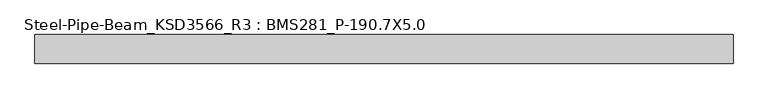
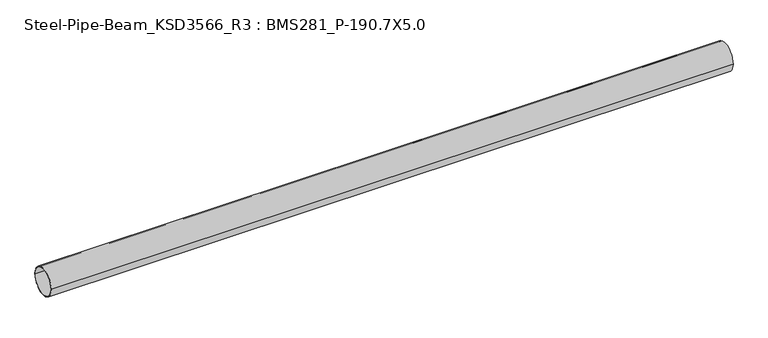
"""IFC4 building model written with IfcOpenShell, lengths in millimetres: member geometry, Steel-Pipe-Beam_KSD3566_R3 : BMS281_P-190.7X5.0."""

from ifc_helpers import new_model, si_unit, point, frame, origin, origin_2d, place, context, project, spatial, circle_curve, trimmed, segment, composite_curve, outline, extrude, source, transform, mapped, element, save


def steel_pipe_beam_ksd3566_r3_bms281_p_190_7x5_0_96b81fe0(model_context):
    return source(origin(), model_context, "Body", "SweptSolid", [
        extrude(outline(composite_curve([segment(trimmed(circle_curve(origin_2d(), 95.35), [point((-95.35, 0.0))], [point((95.35, 0.0))], False, "CARTESIAN"), True, "CONTINUOUS"), segment(trimmed(circle_curve(origin_2d(), 95.35), [point((95.35, 0.0))], [point((-95.35, 0.0))], False, "CARTESIAN"), True, "CONTINUOUS")], self_intersect=False), holes=[composite_curve([segment(trimmed(circle_curve(origin_2d(), 90.35), [point((90.35, 0.0))], [point((-90.35, 0.0))], True, "CARTESIAN"), True, "CONTINUOUS"), segment(trimmed(circle_curve(origin_2d(), 90.35), [point((-90.35, 0.0))], [point((90.35, 0.0))], True, "CARTESIAN"), True, "CONTINUOUS")], self_intersect=False)]), frame((-2303.1049318, 0.0, 0.0), z_axis=(1.0, 0.0, 0.0), x_axis=(0.0, 1.0, 0.0)), (0.0, 0.0, 1.0), 4645.3125185),
    ])


if __name__ == "__main__":
    model = new_model("IFC4")
    model_context = context("Model", 3, world=origin())
    ifc_project = project(units=[si_unit("LENGTHUNIT", "METRE", prefix="MILLI")], contexts=[model_context])
    site = spatial("IfcSite", under=ifc_project)
    building = spatial("IfcBuilding", under=site)
    placement = place(None, origin())
    steel_pipe_beam_ksd3566_r3_bms281_p_190_7x5_0_shape = steel_pipe_beam_ksd3566_r3_bms281_p_190_7x5_0_96b81fe0(model_context)
    element("IfcMember", 1, ObjectType="Steel-Pipe-Beam_KSD3566_R3 : BMS281_P-190.7X5.0", at=placement, inside=building, context=model_context, shape_type="MappedRepresentation", body=[
        mapped(steel_pipe_beam_ksd3566_r3_bms281_p_190_7x5_0_shape, transform((0.0, 0.0, 0.0), x_axis=(1.0, 0.0, 0.0), y_axis=(0.0, 1.0, 0.0), z_axis=(0.0, 0.0, 1.0))),
    ])
    save(model, "model.ifc")

# Revit data of these elements
# Type "Steel-Pipe-Beam_KSD3566_R3 : BMS281_P-190.7X5.0"
#   Keynote = "P-190.7X5.0"
#   SteelWeight = "Light"
#   t = 0.0050 m
#   Surface Area = 0.599102 m²/m
#   Section Area = 29.1697 cm²
#   Mass per Unit Length = 22.8982 kg/m
#   Length [instance default] = 1.5000 m
#   D = 0.1907 m
#   hec_material4 [instance default] = none
#   hec_material3 [instance default] = none
#   hec_material2 [instance default] = none
#   hec_material1 [instance default] = none
#   Structural Material [instance default] = Steel, 45-345
#   Assembly Code = ""
# Element 1 (IfcMember, "Steel-Pipe-Beam_KSD3566_R3 : BMS281_P-190.7X5.0")
#   Structural Material = none
# Materials
#   "Steel, 45-345": class "Metal", colour RGB 189 187 185, transparency 0, Description = "Steel 345 MPa", Cost = 0
